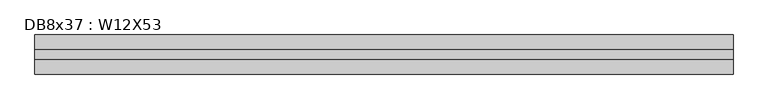
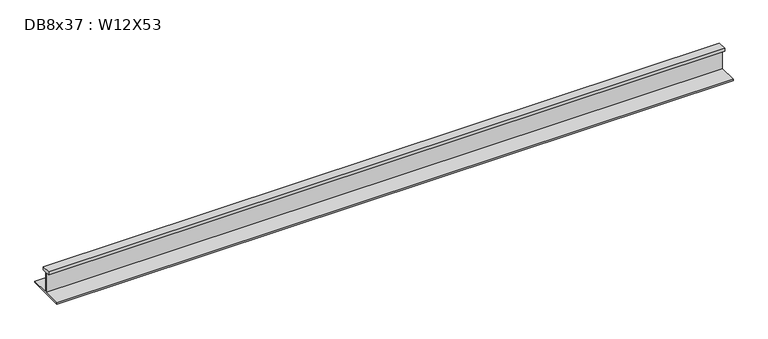
"""IFC4 building model written with IfcOpenShell, lengths in millimetres: beam geometry, DB8x37 : W12X53."""

from ifc_helpers import new_model, si_unit, frame, origin, place, context, project, spatial, polyline, outline, extrude, source, transform, mapped, element, save


def db8x37_w12x53_290fb896(model_context):
    return source(origin(), model_context, "Body", "SweptSolid", [
        extrude(outline(polyline([(38.1, 145.415), (38.1, 120.015), (2.921, 120.015), (2.921, -48.4505), (152.4, -48.4505), (152.4, -58.1025), (-152.4, -58.1025), (-152.4, -48.4505), (-2.921, -48.4505), (-2.921, 120.015), (-38.1, 120.015), (-38.1, 145.415), (38.1, 145.415)])), frame((-2731.008, 0.0, 0.0), z_axis=(1.0, 0.0, 0.0), x_axis=(0.0, 1.0, 0.0)), (0.0, 0.0, 1.0), 5439.537),
    ])


if __name__ == "__main__":
    model = new_model("IFC4")
    model_context = context("Model", 3, world=origin())
    ifc_project = project(units=[si_unit("LENGTHUNIT", "METRE", prefix="MILLI")], contexts=[model_context])
    site = spatial("IfcSite", under=ifc_project)
    building = spatial("IfcBuilding", under=site)
    placement = place(None, origin())
    db8x37_w12x53_shape = db8x37_w12x53_290fb896(model_context)
    element("IfcBeam", 1, ObjectType="DB8x37 : W12X53", at=placement, inside=building, context=model_context, shape_type="MappedRepresentation", body=[
        mapped(db8x37_w12x53_shape, transform((0.0, 0.0, 0.0), x_axis=(1.0, 0.0, 0.0), y_axis=(0.0, 1.0, 0.0), z_axis=(0.0, 0.0, 1.0))),
    ])
    save(model, "model.ifc")

# Revit data of these elements
# Type "DB8x37 : W12X53"
#   Assembly Code = "B10"
#   W = 53
#   Length [instance default] = 5' - 0"
#   bf = 0' - 10"
#   d = 1' - 0.1"
#   k = 0' - 1 3/8"
#   k2 = 0' - 0.8"
#   tf = 0' - 0.575"
#   tw = 0' - 0.345"
#   A = 0.108333 SF
#   Structural Material [instance default] = Steel ASTM A992
# Element 1 (IfcBeam, "DB8x37 : W12X53")
#   Materials on its faces: "Steel ASTM A992"
# Materials
#   "Steel ASTM A992": class "Metal", colour RGB 199 199 199, transparency 0, Description = "Structural steel 50ksi", Cost = 0
